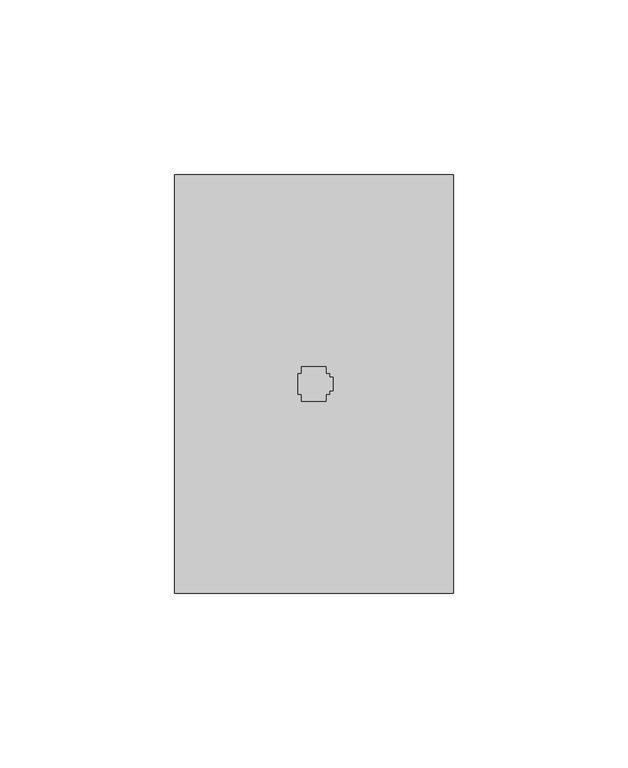
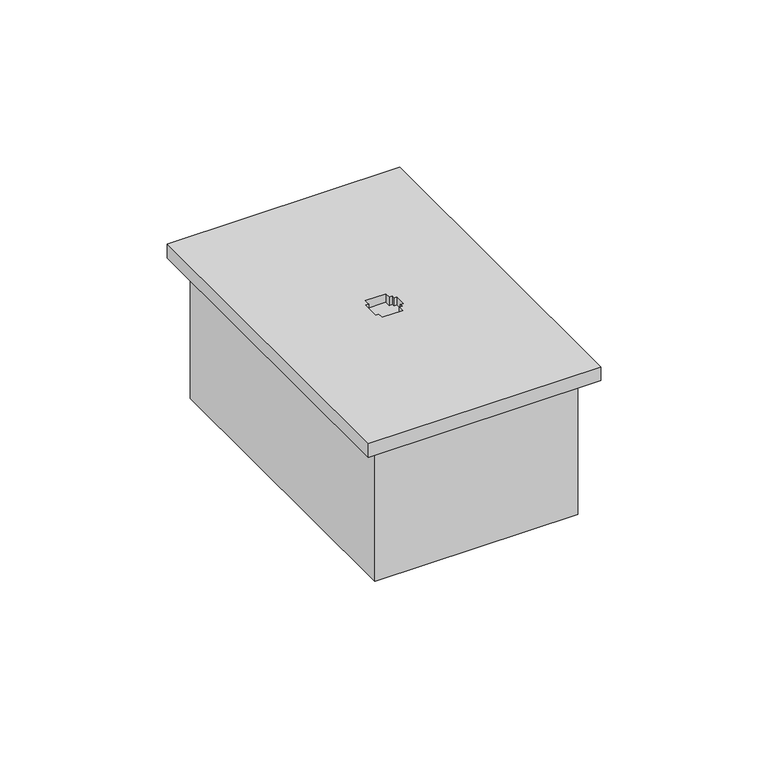
"""IFC4 building model written with IfcOpenShell, lengths in millimetres: proxy geometry, CAIXA VERTICE V7 : Telefone."""

from ifc_helpers import new_model, si_unit, origin, place, context, project, spatial, faceted_brep, source, transform, mapped, element, save


def electrical_fixtures_6f2a964e(model_context):
    return source(origin(), model_context, "Body", "Brep", [
        faceted_brep([(33.0, -1047.0, -48.0), (-33.0, -1047.0, -48.0), (-33.0, -1153.0, -48.0), (33.0, -1153.0, -48.0), (35.0, -1155.0, -50.0), (-35.0, -1155.0, -50.0), (-35.0, -1045.0, -50.0), (35.0, -1045.0, -50.0), (35.0, -1155.0, 0.0), (-35.0, -1155.0, 0.0), (-35.0, -1045.0, 0.0), (35.0, -1045.0, 0.0), (33.0, -1153.0, 0.0), (-33.0, -1153.0, 0.0), (-33.0, -1047.0, 0.0), (33.0, -1047.0, 0.0)], [[[0, 1, 2, 3]], [[4, 5, 6, 7]], [[4, 8, 9, 5]], [[9, 10, 6, 5]], [[10, 11, 7, 6]], [[11, 8, 4, 7]], [[8, 11, 10, 9], [12, 13, 14, 15]], [[15, 0, 3, 12]], [[14, 1, 0, 15]], [[13, 2, 1, 14]], [[12, 3, 2, 13]]]),
        faceted_brep([(40.0, -1160.0, 5.0), (40.0, -1040.0, 5.0), (-40.0, -1040.0, 5.0), (-40.0, -1160.0, 5.0), (-3.5, -1103.0, 5.0), (-4.5, -1103.0, 5.0), (-4.5, -1097.0, 5.0), (-3.5, -1097.0, 5.0), (-3.5, -1095.0, 5.0), (3.5, -1095.0, 5.0), (3.5, -1097.0, 5.0), (4.5, -1097.0, 5.0), (4.5, -1098.0, 5.0), (5.5, -1098.0, 5.0), (5.5, -1102.0, 5.0), (4.5, -1102.0, 5.0), (4.5, -1103.0, 5.0), (3.5, -1103.0, 5.0), (3.5, -1105.0, 5.0), (-3.5, -1105.0, 5.0), (-40.0, -1160.0, 0.0), (-40.0, -1040.0, 0.0), (40.0, -1040.0, 0.0), (40.0, -1160.0, 0.0), (-3.5, -1103.0, 2.0), (-3.5, -1105.0, 2.0), (-4.5, -1103.0, 2.0), (-4.5, -1097.0, 2.0), (-3.5, -1097.0, 2.0), (-3.5, -1095.0, 2.0), (3.5, -1095.0, 2.0), (3.5, -1097.0, 2.0), (3.5, -1105.0, 2.0), (3.5, -1103.0, 2.0), (4.5, -1103.0, 2.0), (4.5, -1102.0, 2.0), (5.5, -1102.0, 2.0), (5.5, -1098.0, 2.0), (4.5, -1098.0, 2.0), (4.5, -1097.0, 2.0)], [[[0, 1, 2, 3], [4, 5, 6, 7, 8, 9, 10, 11, 12, 13, 14, 15, 16, 17, 18, 19]], [[20, 21, 22, 23]], [[3, 20, 23, 0]], [[2, 21, 20, 3]], [[1, 22, 21, 2]], [[0, 23, 22, 1]], [[24, 4, 19, 25]], [[26, 5, 4, 24]], [[27, 6, 5, 26]], [[28, 7, 6, 27]], [[29, 8, 7, 28]], [[30, 9, 8, 29]], [[31, 10, 9, 30]], [[32, 33, 34, 35, 36, 37, 38, 39, 31, 30, 29, 28, 27, 26, 24, 25]], [[25, 19, 18, 32]], [[39, 11, 10, 31]], [[38, 12, 11, 39]], [[37, 13, 12, 38]], [[36, 14, 13, 37]], [[35, 15, 14, 36]], [[34, 16, 15, 35]], [[33, 17, 16, 34]], [[32, 18, 17, 33]]]),
    ])


if __name__ == "__main__":
    model = new_model("IFC4")
    model_context = context("Model", 3, world=origin())
    ifc_project = project(units=[si_unit("LENGTHUNIT", "METRE", prefix="MILLI")], contexts=[model_context])
    site = spatial("IfcSite", under=ifc_project)
    building = spatial("IfcBuilding", under=site)
    placement = place(None, origin())
    electrical_fixtures_shape = electrical_fixtures_6f2a964e(model_context)
    element("IfcBuildingElementProxy", 1, Name="CAIXA VERTICE V7 : Telefone", ObjectType="CAIXA VERTICE V7 : Telefone", at=placement, inside=building, context=model_context, shape_type="MappedRepresentation", body=[
        mapped(electrical_fixtures_shape, transform((0.0, 0.0, 0.0), x_axis=(1.0, 0.0, 0.0), y_axis=(0.0, 1.0, 0.0), z_axis=(0.0, 0.0, 1.0))),
    ])
    save(model, "model.ifc")

# Revit data of these elements
# Type "CAIXA VERTICE V7 : Telefone"
#   URL = "www.facebook.com/verticetreinamentos"
#   SEÇÃO [instance default] = ""
#   Rotação [instance default] = 0.00°
#   LARGURA DA TAMPA = 0.08 m
#   BORDA = 0.01 m
#   ALTURA DE INSTALAÇÃO [instance default] = 1.10 m
#   Distância Anotação [instance default] = 0.0015 m
#   ALTURA DA TAMPA = 0.12 m
#   Vertical [instance default] = yes
#   VER SEÇÃO [instance default] = no
#   SHADE ESQ [instance default] = no
#   SHADE DIR [instance default] = yes
#   HORIZONTAL [instance default] = no
#   ANDAR COM A LEGENDA [instance default] = 0
#   Material Tampa [instance default] = Plástico, branco opaco
#   Caixa = element 1798520
#   Anotação = element 1798519
#   Default Elevation = 0
# Element 1 (IfcBuildingElementProxy, "CAIXA VERTICE V7 : Telefone")
#   VER SEÇÃO = yes
#   Materials on its faces: "Plástico, branco opaco"
# Materials
#   "Plástico, branco opaco": class "Plástico", colour RGB 120 120 120, transparency 0, Description = "Plastic, generic, opaque white", Cost = 0
